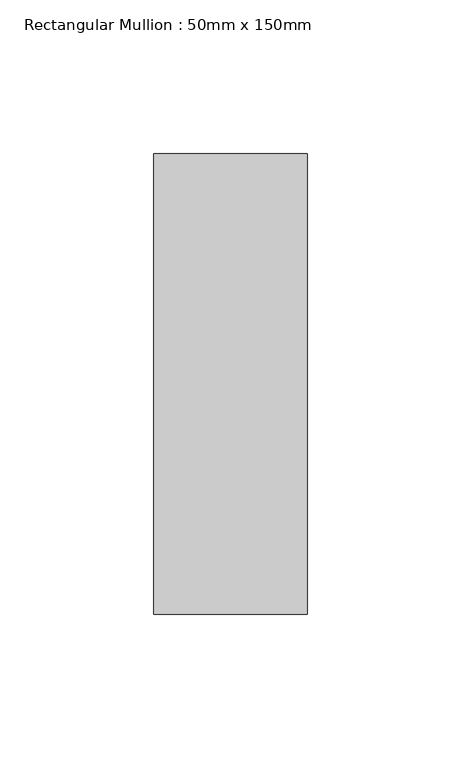
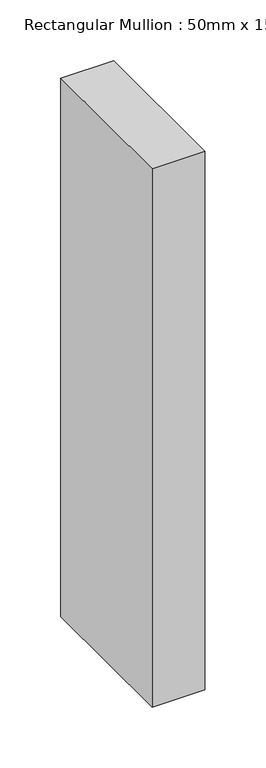
"""IFC4 building model written with IfcOpenShell, lengths in millimetres: member geometry, Rectangular Mullion : 50mm x 150mm."""

from ifc_helpers import new_model, si_unit, frame, origin, place, context, project, spatial, polyline, outline, extrude, source, transform, mapped, element, save


def rectangular_mullion_50mm_x_150mm_8f37db85(model_context):
    return source(origin(), model_context, "Body", "SweptSolid", [
        extrude(outline(polyline([(0.0, 75.0), (0.0, -75.0), (-50.0, -75.0), (-50.0, 75.0), (0.0, 75.0)])), frame((0.0, 0.0, -540.0), z_axis=(0.0, 0.0, 1.0), x_axis=(1.0, 0.0, 0.0)), (0.0, 0.0, 1.0), 540.0),
    ])


if __name__ == "__main__":
    model = new_model("IFC4")
    model_context = context("Model", 3, world=origin())
    ifc_project = project(units=[si_unit("LENGTHUNIT", "METRE", prefix="MILLI")], contexts=[model_context])
    site = spatial("IfcSite", under=ifc_project)
    building = spatial("IfcBuilding", under=site)
    placement = place(None, origin())
    rectangular_mullion_50mm_x_150mm_shape = rectangular_mullion_50mm_x_150mm_8f37db85(model_context)
    element("IfcMember", 1, ObjectType="Rectangular Mullion : 50mm x 150mm", at=placement, inside=building, context=model_context, shape_type="MappedRepresentation", body=[
        mapped(rectangular_mullion_50mm_x_150mm_shape, transform((0.0, 0.0, 0.0), x_axis=(1.0, 0.0, 0.0), y_axis=(0.0, 1.0, 0.0), z_axis=(0.0, 0.0, 1.0))),
    ])
    save(model, "model.ifc")

# Revit data of these elements
# Type "Rectangular Mullion : 50mm x 150mm"
#   built-in parameter 1007304 = 0.492126 (stored number, unit not read)
#   built-in parameter 1007301 = 0.082021 (stored number, unit not read)
#   built-in parameter 1007300 = 0.082021 (stored number, unit not read)
# Element 1 (IfcMember, "Rectangular Mullion : 50mm x 150mm")
#   Materials on its faces: "Aluminum"
# Materials
#   "Aluminum": class "Metal", colour RGB 244 244 244, transparency 0, Description = "Aluminum 6061", Cost = 0
